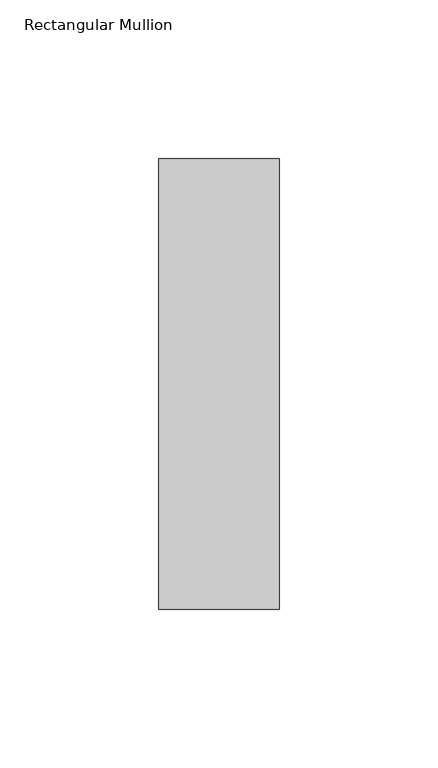
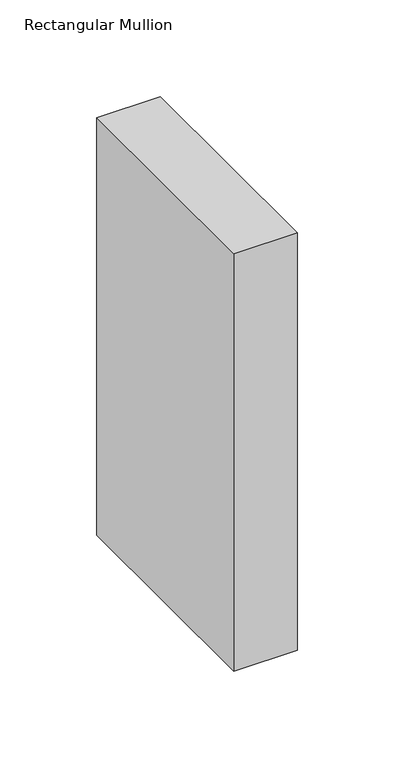
"""IFC4 building model written with IfcOpenShell, lengths in millimetres: member geometry, Rectangular Mullion : NLRS_21_CWM_hsb-regel 38x142_gen_rsf."""

from ifc_helpers import new_model, si_unit, frame, origin, place, context, project, spatial, polyline, outline, extrude, source, transform, mapped, element, save


def rectangular_mullion_45174ede(model_context):
    return source(origin(), model_context, "Body", "SweptSolid", [
        extrude(outline(polyline([(0.0, -71.0), (-38.0, -71.0), (-38.0, 71.0), (0.0, 71.0), (0.0, -71.0)])), frame((0.0, 0.0, -264.0000003), z_axis=(0.0, 0.0, 1.0), x_axis=(1.0, 0.0, 0.0)), (0.0, 0.0, 1.0), 264.0000003),
    ])


if __name__ == "__main__":
    model = new_model("IFC4")
    model_context = context("Model", 3, world=origin())
    ifc_project = project(units=[si_unit("LENGTHUNIT", "METRE", prefix="MILLI")], contexts=[model_context])
    site = spatial("IfcSite", under=ifc_project)
    building = spatial("IfcBuilding", under=site)
    placement = place(None, origin())
    rectangular_mullion_shape = rectangular_mullion_45174ede(model_context)
    element("IfcMember", 1, ObjectType="Rectangular Mullion : NLRS_21_CWM_hsb-regel 38x142_gen_rsf", at=placement, inside=building, context=model_context, shape_type="MappedRepresentation", body=[
        mapped(rectangular_mullion_shape, transform((0.0, 0.0, 0.0), x_axis=(1.0, 0.0, 0.0), y_axis=(0.0, 1.0, 0.0), z_axis=(0.0, 0.0, 1.0))),
    ])
    save(model, "model.ifc")

# Revit data of these elements
# Type "Rectangular Mullion : NLRS_21_CWM_hsb-regel 38x142_gen_rsf"
#   Export Type to IFC As = "IfcWall"
#   Type IfcGUID = "07M7mRoiH1CR8m_RSKIwpF"
#   Assembly Code = "21.10"
#   built-in parameter 1007322 = 0.465879 (stored number, unit not read)
#   built-in parameter 1007321 = 0.062336 (stored number, unit not read)
#   built-in parameter 1007320 = 0.062336 (stored number, unit not read)
# Element 1 (IfcMember, "Rectangular Mullion : NLRS_21_CWM_hsb-regel 38x142_gen_rsf")
#   Materials on its faces: "NLRS_i2_hout naaldhout vuren_gen_rsf"
# Materials
#   "NLRS_i2_hout naaldhout vuren_gen_rsf": class "I - Hout", colour RGB 234 199 147, transparency 0, Keynote = "i2", Manufacturer = "Revit Standards Foundation", URL = "www.revitstandards.org", Description = "hout vuren", Cost = 0
